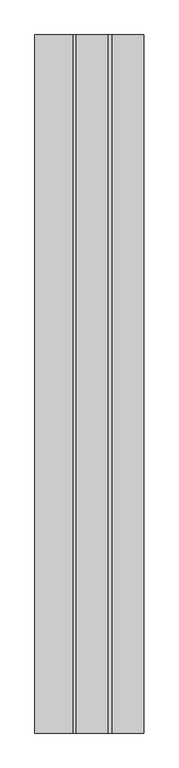
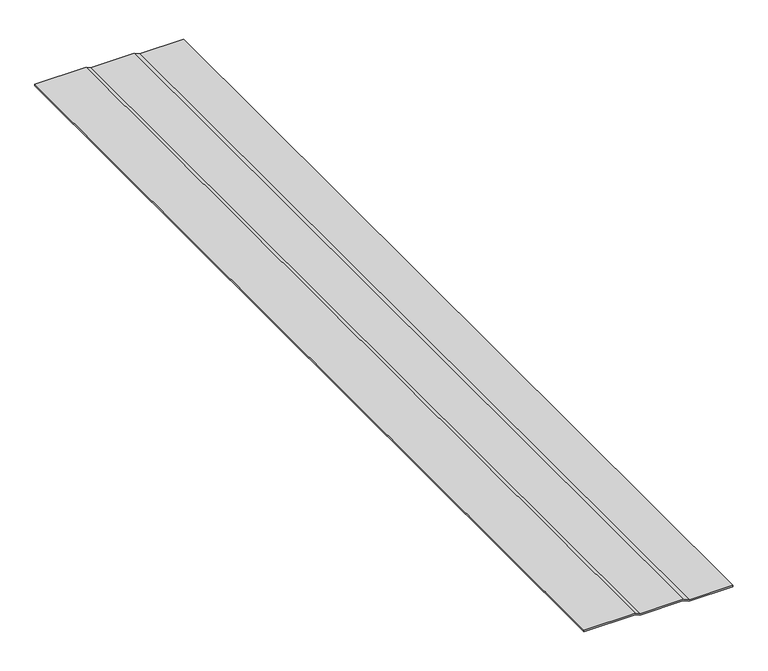
"""IFC4 building model written with IfcOpenShell, lengths in millimetres: proxy geometry, BITUMEN CAP SHEET3:BITUMEN CAP SHEET001:300094 : BITUMEN CAP SHEET3:BITUMEN CAP SHEET001:300094."""

from ifc_helpers import new_model, si_unit, frame, origin, place, context, project, spatial, polyline, outline, extrude, source, transform, mapped, element, save


def generic_models_9b3239e1(model_context):
    return source(origin(), model_context, "Body", "SweptSolid", [
        extrude(outline(polyline([(40259.2002678, -14.96193), (40259.2002678, 77.2027316), (40262.3752679, 77.2027316), (40262.3752679, -14.31653), (40267.6612773, -26.7813486), (40267.6612773, -117.4651043), (40271.994072, -127.1820058), (40271.994072, -235.0685024), (40268.8188423, -235.0685024), (40268.8188423, -127.8572913), (40264.4862773, -118.1409048), (40264.4862773, -27.4267486), (40259.2002678, -14.96193)])), frame((0.0, -774.5581163, 0.0), z_axis=(0.0, 1.0, 0.0), x_axis=(0.0, 0.0, 1.0)), (0.0, 0.0, 1.0), 2000.25),
    ])


if __name__ == "__main__":
    model = new_model("IFC4")
    model_context = context("Model", 3, world=origin())
    ifc_project = project(units=[si_unit("LENGTHUNIT", "METRE", prefix="MILLI")], contexts=[model_context])
    site = spatial("IfcSite", under=ifc_project)
    building = spatial("IfcBuilding", under=site)
    placement = place(None, origin())
    generic_models_shape = generic_models_9b3239e1(model_context)
    element("IfcBuildingElementProxy", 1, Name="BITUMEN CAP SHEET3:BITUMEN CAP SHEET001:300094 : BITUMEN CAP SHEET3:BITUMEN CAP SHEET001:300094", ObjectType="BITUMEN CAP SHEET3:BITUMEN CAP SHEET001:300094 : BITUMEN CAP SHEET3:BITUMEN CAP SHEET001:300094", at=placement, inside=building, context=model_context, shape_type="MappedRepresentation", body=[
        mapped(generic_models_shape, transform((0.0, 0.0, 0.0), x_axis=(1.0, 0.0, 0.0), y_axis=(0.0, 1.0, 0.0), z_axis=(0.0, 0.0, 1.0))),
    ])
    save(model, "model.ifc")

# Revit data of these elements
# Type "BITUMEN CAP SHEET3:BITUMEN CAP SHEET001:300094 : BITUMEN CAP SHEET3:BITUMEN CAP SHEET001:300094"
#   NameOverride = "BITUMEN CAP SHEET3:BITUMEN CAP SHEET001:300094"
#   ObjectTypeOverride = "BITUMEN CAP SHEET3:BITUMEN CAP SHEET001"
#   Reference = "BITUMEN CAP SHEET001"
#   Category = "Generic Models"
#   Tag = "300094"
# Element 1 (IfcBuildingElementProxy, "BITUMEN CAP SHEET3:BITUMEN CAP SHEET001:300094 : BITUMEN CAP SHEET3:BITUMEN CAP SHEET001:300094")
#   Materials on its faces: "MODIFIED BITUMEN GRANULE SURFACED CAP SHEET"
# Materials
#   "MODIFIED BITUMEN GRANULE SURFACED CAP SHEET": class "Unassigned", colour RGB 85 85 127, transparency 0
